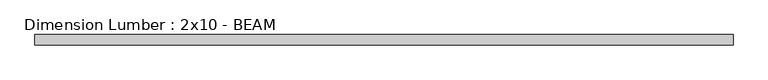
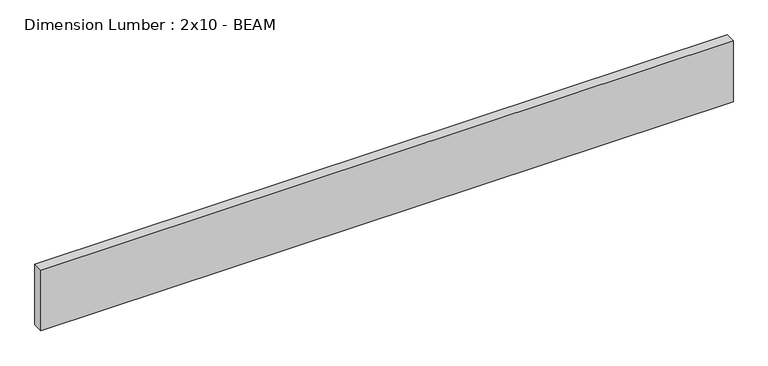
"""IFC4 building model written with IfcOpenShell, lengths in millimetres: beam geometry, Dimension Lumber : 2x10 - BEAM."""

from ifc_helpers import new_model, si_unit, frame, origin, place, context, project, spatial, polyline, outline, extrude, source, transform, mapped, element, save


def dimension_lumber_2x10_beam_c9fcd336(model_context):
    return source(origin(), model_context, "Body", "SweptSolid", [
        extrude(outline(polyline([(1212.1306641, 19.05), (1212.1306641, -19.05), (-1321.214473, -19.05), (-1321.214473, 19.05), (1212.1306641, 19.05)])), frame((0.0, 0.0, -117.475), z_axis=(0.0, 0.0, 1.0), x_axis=(1.0, 0.0, 0.0)), (0.0, 0.0, 1.0), 234.95),
    ])


if __name__ == "__main__":
    model = new_model("IFC4")
    model_context = context("Model", 3, world=origin())
    ifc_project = project(units=[si_unit("LENGTHUNIT", "METRE", prefix="MILLI")], contexts=[model_context])
    site = spatial("IfcSite", under=ifc_project)
    building = spatial("IfcBuilding", under=site)
    placement = place(None, origin())
    dimension_lumber_2x10_beam_shape = dimension_lumber_2x10_beam_c9fcd336(model_context)
    element("IfcBeam", 1, ObjectType="Dimension Lumber : 2x10 - BEAM", at=placement, inside=building, context=model_context, shape_type="MappedRepresentation", body=[
        mapped(dimension_lumber_2x10_beam_shape, transform((0.0, 0.0, 0.0), x_axis=(1.0, 0.0, 0.0), y_axis=(0.0, 1.0, 0.0), z_axis=(0.0, 0.0, 1.0))),
    ])
    save(model, "model.ifc")

# Revit data of these elements
# Type "Dimension Lumber : 2x10 - BEAM"
#   Assembly Code = "B10"
#   A = 0.0755556 SF
#   Length [instance default] = 5' - 0"
#   b = 0' - 1 1/2"
#   d = 0' - 9 1/4"
#   Structural Material = (3) SISTERED 2X10s AT BEAM
# Element 1 (IfcBeam, "Dimension Lumber : 2x10 - BEAM")
#   Materials on its faces: "(3) SISTERED 2X10s AT BEAM"
# Materials
#   "(3) SISTERED 2X10s AT BEAM": class "Wood", colour RGB 234 198 147, transparency 0, Description = "Pinus Echinata", Cost = 0
